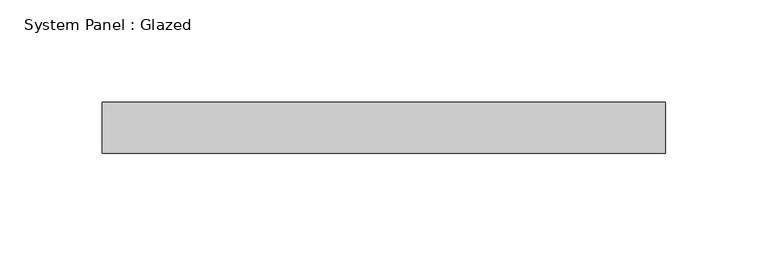
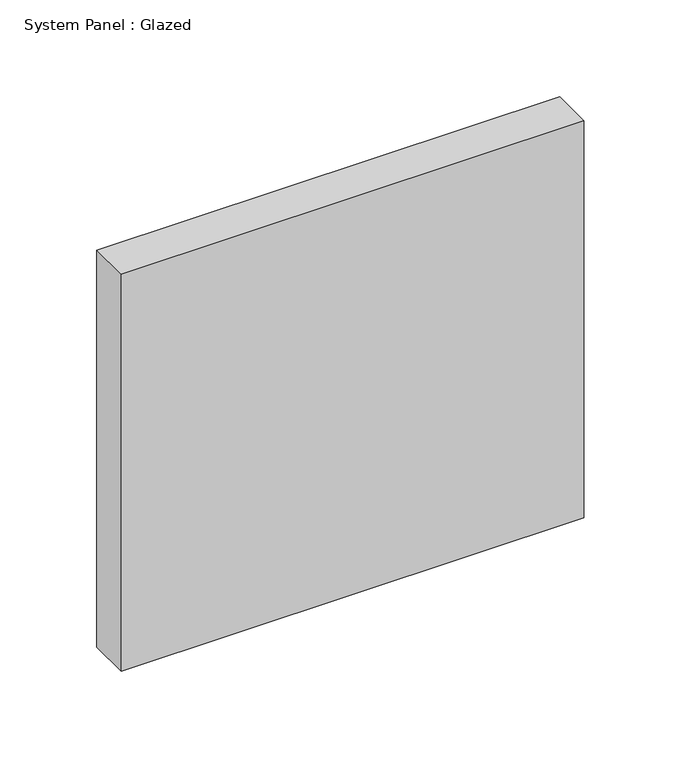
"""IFC4 building model written with IfcOpenShell, lengths in millimetres: plate geometry, System Panel : Glazed."""

from ifc_helpers import new_model, si_unit, origin, origin_with_axes, place, context, project, spatial, polyline, outline, extrude, source, transform, mapped, element, save


def system_panel_glazed_1635d049(model_context):
    return source(origin(), model_context, "Body", "SweptSolid", [
        extrude(outline(polyline([(137.8787879, 24.5), (-137.8787879, 24.5), (-137.8787879, 49.5), (137.8787879, 49.5), (137.8787879, 24.5)])), origin_with_axes(), (0.0, 0.0, 1.0), 250.0),
    ])


if __name__ == "__main__":
    model = new_model("IFC4")
    model_context = context("Model", 3, world=origin())
    ifc_project = project(units=[si_unit("LENGTHUNIT", "METRE", prefix="MILLI")], contexts=[model_context])
    site = spatial("IfcSite", under=ifc_project)
    building = spatial("IfcBuilding", under=site)
    placement = place(None, origin())
    system_panel_glazed_shape = system_panel_glazed_1635d049(model_context)
    element("IfcPlate", 1, ObjectType="System Panel : Glazed", at=placement, inside=building, context=model_context, shape_type="MappedRepresentation", body=[
        mapped(system_panel_glazed_shape, transform((0.0, 0.0, 0.0), x_axis=(1.0, 0.0, 0.0), y_axis=(0.0, 1.0, 0.0), z_axis=(0.0, 0.0, 1.0))),
    ])
    save(model, "model.ifc")

# Revit data of these elements
# Element 1 (IfcPlate, "System Panel : Glazed")
#   Materials on its faces: "Glass"
# Materials
#   "Glass": class "Glass", colour RGB 218 227 224, transparency 0.85, Description = "Soda Lime Glass", Cost = 0
